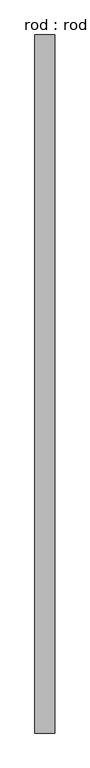
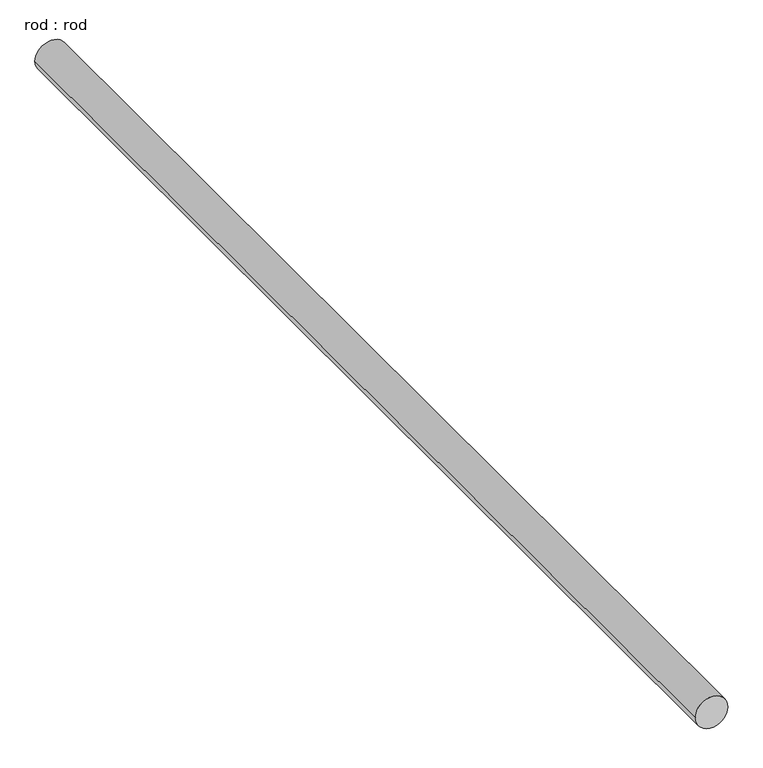
"""IFC4 building model written with IfcOpenShell, lengths in millimetres: proxy geometry, rod : rod."""

from ifc_helpers import new_model, si_unit, point, frame, frame_2d, origin, place, context, project, spatial, circle_curve, trimmed, segment, composite_curve, outline, extrude, source, transform, mapped, element, save


def rod_rod_9554ad8a(model_context):
    return source(origin(), model_context, "Body", "SweptSolid", [
        extrude(outline(composite_curve([segment(trimmed(circle_curve(frame_2d((0.0108462, 0.0)), 200.0), [point((0.0108462, 200.0))], [point((0.0108462, -200.0))], False, "CARTESIAN"), True, "CONTINUOUS"), segment(trimmed(circle_curve(frame_2d((0.0108462, 0.0)), 200.0), [point((0.0108462, -200.0))], [point((0.0108462, 200.0))], False, "CARTESIAN"), True, "CONTINUOUS")], self_intersect=False)), frame((0.0, -2906.1681727, 0.0), z_axis=(0.0, 1.0, 0.0), x_axis=(0.0, 0.0, 1.0)), (0.0, 0.0, 1.0), 13997.7935761),
    ])


if __name__ == "__main__":
    model = new_model("IFC4")
    model_context = context("Model", 3, world=origin())
    ifc_project = project(units=[si_unit("LENGTHUNIT", "METRE", prefix="MILLI")], contexts=[model_context])
    site = spatial("IfcSite", under=ifc_project)
    building = spatial("IfcBuilding", under=site)
    placement = place(None, origin())
    rod_rod_shape = rod_rod_9554ad8a(model_context)
    element("IfcBuildingElementProxy", 1, Name="rod : rod", ObjectType="rod : rod", at=placement, inside=building, context=model_context, shape_type="MappedRepresentation", body=[
        mapped(rod_rod_shape, transform((0.0, 0.0, 0.0), x_axis=(1.0, 0.0, 0.0), y_axis=(0.0, 1.0, 0.0), z_axis=(0.0, 0.0, 1.0))),
    ])
    save(model, "model.ifc")

# Revit data of these elements
# Type "rod : rod"
#   Default Elevation = 0
